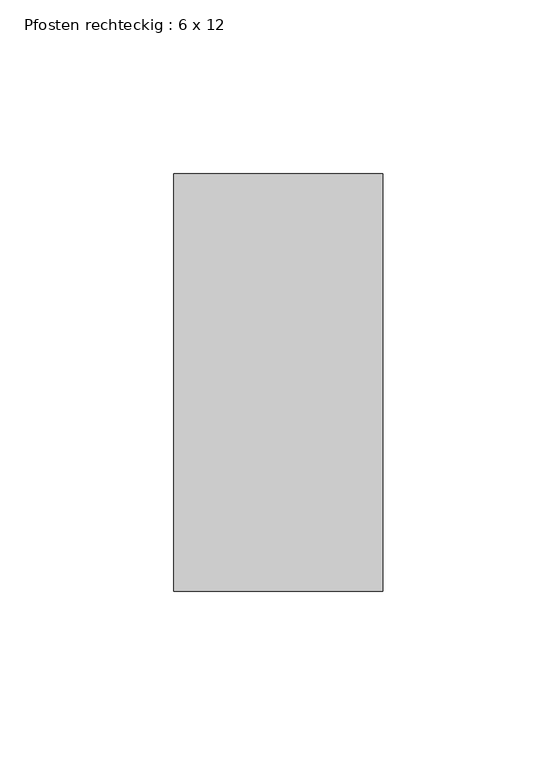
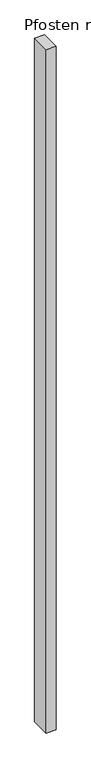
"""IFC4 building model written with IfcOpenShell, lengths in millimetres: member geometry, Pfosten rechteckig : 6 x 12."""

from ifc_helpers import new_model, si_unit, frame, origin, place, context, project, spatial, polyline, outline, extrude, source, transform, mapped, element, save


def pfosten_rechteckig_6_x_12_73fb7427(model_context):
    return source(origin(), model_context, "Body", "SweptSolid", [
        extrude(outline(polyline([(30.0, 60.0), (30.0, -60.0), (-30.0, -60.0), (-30.0, 60.0), (30.0, 60.0)])), frame((0.0, 0.0, -4356.6788019), z_axis=(0.0, 0.0, 1.0), x_axis=(1.0, 0.0, 0.0)), (0.0, 0.0, 1.0), 4356.6788019),
    ])


if __name__ == "__main__":
    model = new_model("IFC4")
    model_context = context("Model", 3, world=origin())
    ifc_project = project(units=[si_unit("LENGTHUNIT", "METRE", prefix="MILLI")], contexts=[model_context])
    site = spatial("IfcSite", under=ifc_project)
    building = spatial("IfcBuilding", under=site)
    placement = place(None, origin())
    pfosten_rechteckig_6_x_12_shape = pfosten_rechteckig_6_x_12_73fb7427(model_context)
    element("IfcMember", 1, ObjectType="Pfosten rechteckig : 6 x 12", at=placement, inside=building, context=model_context, shape_type="MappedRepresentation", body=[
        mapped(pfosten_rechteckig_6_x_12_shape, transform((0.0, 0.0, 0.0), x_axis=(1.0, 0.0, 0.0), y_axis=(0.0, 1.0, 0.0), z_axis=(0.0, 0.0, 1.0))),
    ])
    save(model, "model.ifc")

# Revit data of these elements
# Type "Pfosten rechteckig : 6 x 12"
#   built-in parameter 1007304 = 0.393701 (stored number, unit not read)
#   built-in parameter 1007301 = 0.0984252 (stored number, unit not read)
#   built-in parameter 1007300 = 0.0984252 (stored number, unit not read)
# Element 1 (IfcMember, "Pfosten rechteckig : 6 x 12")
#   Materials on its faces: "Metall - verzinkt"
# Materials
#   "Metall - verzinkt": class "Allgemeines", colour RGB 200 200 200, transparency 0, Cost = 0
